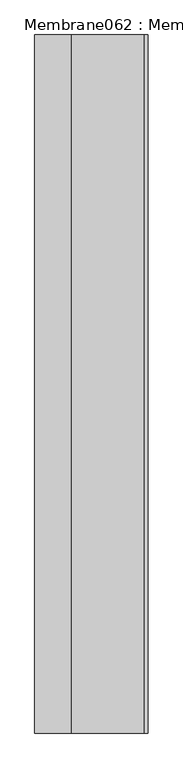
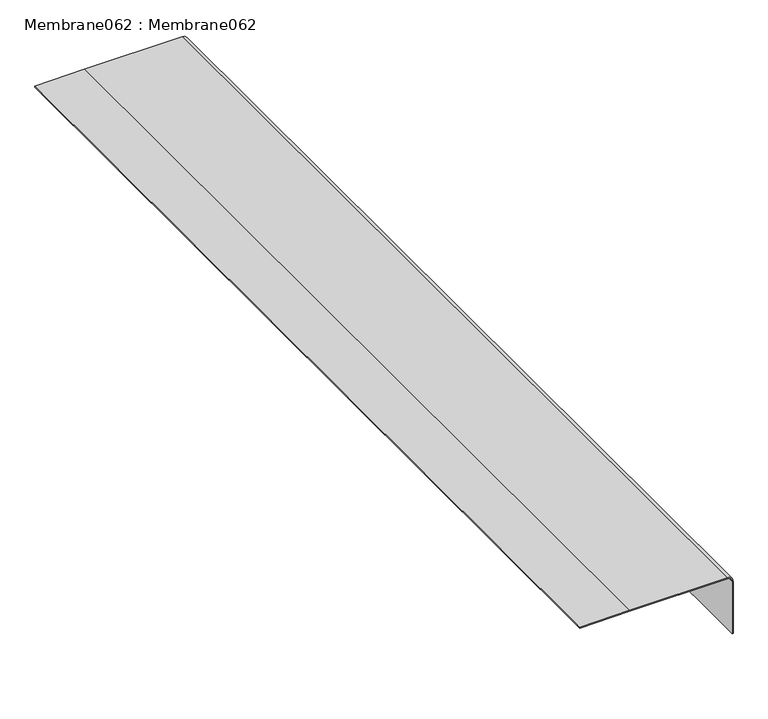
"""IFC4 building model written with IfcOpenShell, lengths in millimetres: proxy geometry, Membrane062 : Membrane062."""

from ifc_helpers import new_model, si_unit, point, frame, frame_2d, origin, place, context, project, spatial, polyline, circle_curve, trimmed, segment, composite_curve, outline, extrude, source, transform, mapped, element, save


def membrane062_membrane062_3a08a67c(model_context):
    return source(origin(), model_context, "Body", "SweptSolid", [
        extrude(outline(composite_curve([segment(polyline([(40233.3001163, -4377.1070699), (40116.5801181, -4377.1070699), (40116.5801181, -4375.1070699), (40233.3001163, -4375.1070699)]), True, "CONTINUOUS"), segment(trimmed(circle_curve(frame_2d((40233.3001163, -4387.1070699)), 12.0), [point((40233.3001163, -4375.1070699))], [point((40245.3001163, -4387.1070699))], False, "CARTESIAN"), True, "CONTINUOUS"), segment(polyline([(40245.3001163, -4387.1070699), (40245.3001163, -4595.4560976), (40243.79743, -4699.8063764), (40241.7972226, -4699.8063764), (40243.3001163, -4595.4416982), (40243.3001163, -4387.1070699)]), True, "CONTINUOUS"), segment(trimmed(circle_curve(frame_2d((40233.3001163, -4387.1070699)), 10.0), [point((40243.3001163, -4387.1070699))], [point((40233.3001163, -4377.1070699))], True, "CARTESIAN"), True, "CONTINUOUS")], self_intersect=False)), frame((0.0, -1052.8906574, 0.0), z_axis=(0.0, 1.0, 0.0), x_axis=(0.0, 0.0, 1.0)), (0.0, 0.0, 1.0), 2000.0),
    ])


if __name__ == "__main__":
    model = new_model("IFC4")
    model_context = context("Model", 3, world=origin())
    ifc_project = project(units=[si_unit("LENGTHUNIT", "METRE", prefix="MILLI")], contexts=[model_context])
    site = spatial("IfcSite", under=ifc_project)
    building = spatial("IfcBuilding", under=site)
    placement = place(None, origin())
    membrane062_membrane062_shape = membrane062_membrane062_3a08a67c(model_context)
    element("IfcBuildingElementProxy", 1, Name="Membrane062 : Membrane062", ObjectType="Membrane062 : Membrane062", at=placement, inside=building, context=model_context, shape_type="MappedRepresentation", body=[
        mapped(membrane062_membrane062_shape, transform((0.0, 0.0, 0.0), x_axis=(1.0, 0.0, 0.0), y_axis=(0.0, 1.0, 0.0), z_axis=(0.0, 0.0, 1.0))),
    ])
    save(model, "model.ifc")

# Revit data of these elements
# Type "Membrane062 : Membrane062"
#   NameOverride = "Membrane062"
# Element 1 (IfcBuildingElementProxy, "Membrane062 : Membrane062")
#   Materials on its faces: "THREE PLY BUILT UP ROOF MEMBRANE"
# Materials
#   "THREE PLY BUILT UP ROOF MEMBRANE": class "Unassigned", colour RGB 63 63 63, transparency 0
